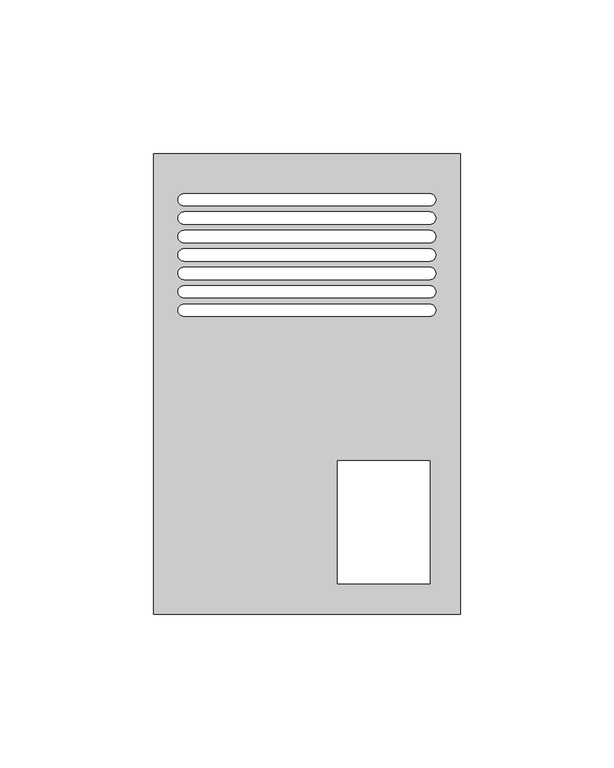
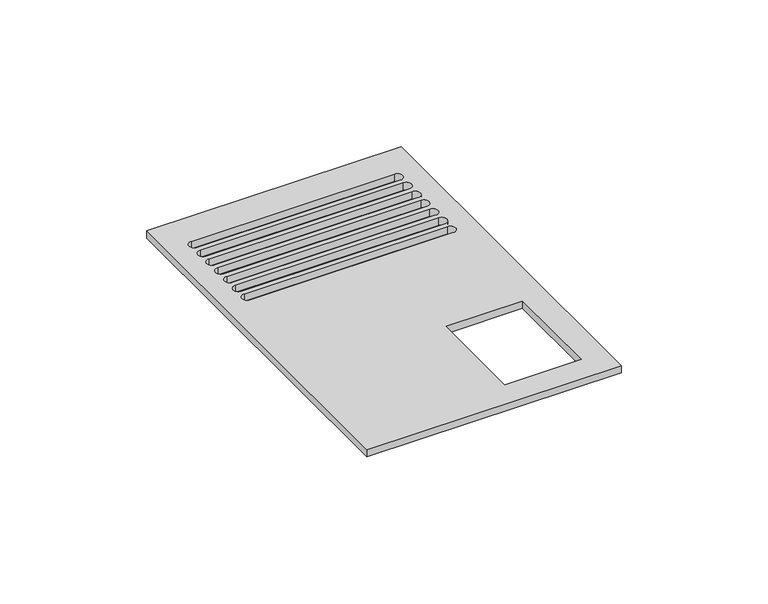
"""IFC4 building model written with IfcOpenShell, lengths in millimetres: proxy geometry, TSP Intercom Point : TSP Intercom Point."""

from ifc_helpers import new_model, si_unit, point, frame_2d, origin, origin_with_axes, place, context, project, spatial, polyline, circle_curve, trimmed, segment, composite_curve, outline, extrude, source, transform, mapped, element, save


def electrical_fixtures_fec92b32(model_context):
    return source(origin(), model_context, "Body", "SweptSolid", [
        extrude(outline(polyline([(-100.0, 75.0), (0.0, 75.0), (0.0, -75.0), (-100.0, -75.0), (-100.0, 75.0)]), holes=[polyline([(-40.0, -65.0), (-10.0, -65.0), (-10.0, -25.0), (-40.0, -25.0), (-40.0, -65.0)]), composite_curve([segment(polyline([(-10.0, 62.0), (-90.0, 62.0)]), True, "CONTINUOUS"), segment(trimmed(circle_curve(frame_2d((-90.0, 60.0)), 2.0), [point((-90.0, 62.0))], [point((-90.0, 58.0))], True, "CARTESIAN"), True, "CONTINUOUS"), segment(polyline([(-90.0, 58.0), (-10.0, 58.0)]), True, "CONTINUOUS"), segment(trimmed(circle_curve(frame_2d((-10.0, 60.0)), 2.0), [point((-10.0, 58.0))], [point((-10.0, 62.0))], True, "CARTESIAN"), True, "CONTINUOUS")], self_intersect=False), composite_curve([segment(polyline([(-10.0, 56.0), (-90.0, 56.0)]), True, "CONTINUOUS"), segment(trimmed(circle_curve(frame_2d((-90.0, 54.0)), 2.0), [point((-90.0, 56.0))], [point((-90.0, 52.0))], True, "CARTESIAN"), True, "CONTINUOUS"), segment(polyline([(-90.0, 52.0), (-10.0, 52.0)]), True, "CONTINUOUS"), segment(trimmed(circle_curve(frame_2d((-10.0, 54.0)), 2.0), [point((-10.0, 52.0))], [point((-10.0, 56.0))], True, "CARTESIAN"), True, "CONTINUOUS")], self_intersect=False), composite_curve([segment(polyline([(-10.0, 50.0), (-90.0, 50.0)]), True, "CONTINUOUS"), segment(trimmed(circle_curve(frame_2d((-90.0, 48.0)), 2.0), [point((-90.0, 50.0))], [point((-90.0, 46.0))], True, "CARTESIAN"), True, "CONTINUOUS"), segment(polyline([(-90.0, 46.0), (-10.0, 46.0)]), True, "CONTINUOUS"), segment(trimmed(circle_curve(frame_2d((-10.0, 48.0)), 2.0), [point((-10.0, 46.0))], [point((-10.0, 50.0))], True, "CARTESIAN"), True, "CONTINUOUS")], self_intersect=False), composite_curve([segment(polyline([(-10.0, 44.0), (-90.0, 44.0)]), True, "CONTINUOUS"), segment(trimmed(circle_curve(frame_2d((-90.0, 42.0)), 2.0), [point((-90.0, 44.0))], [point((-90.0, 40.0))], True, "CARTESIAN"), True, "CONTINUOUS"), segment(polyline([(-90.0, 40.0), (-10.0, 40.0)]), True, "CONTINUOUS"), segment(trimmed(circle_curve(frame_2d((-10.0, 42.0)), 2.0), [point((-10.0, 40.0))], [point((-10.0, 44.0))], True, "CARTESIAN"), True, "CONTINUOUS")], self_intersect=False), composite_curve([segment(polyline([(-10.0, 38.0), (-90.0, 38.0)]), True, "CONTINUOUS"), segment(trimmed(circle_curve(frame_2d((-90.0, 36.0)), 2.0), [point((-90.0, 38.0))], [point((-90.0, 34.0))], True, "CARTESIAN"), True, "CONTINUOUS"), segment(polyline([(-90.0, 34.0), (-10.0, 34.0)]), True, "CONTINUOUS"), segment(trimmed(circle_curve(frame_2d((-10.0, 36.0)), 2.0), [point((-10.0, 34.0))], [point((-10.0, 38.0))], True, "CARTESIAN"), True, "CONTINUOUS")], self_intersect=False), composite_curve([segment(polyline([(-10.0, 32.0), (-90.0, 32.0)]), True, "CONTINUOUS"), segment(trimmed(circle_curve(frame_2d((-90.0, 30.0)), 2.0), [point((-90.0, 32.0))], [point((-90.0, 28.0))], True, "CARTESIAN"), True, "CONTINUOUS"), segment(polyline([(-90.0, 28.0), (-10.0, 28.0)]), True, "CONTINUOUS"), segment(trimmed(circle_curve(frame_2d((-10.0, 30.0)), 2.0), [point((-10.0, 28.0))], [point((-10.0, 32.0))], True, "CARTESIAN"), True, "CONTINUOUS")], self_intersect=False), composite_curve([segment(polyline([(-10.0, 26.0), (-90.0, 26.0)]), True, "CONTINUOUS"), segment(trimmed(circle_curve(frame_2d((-90.0, 24.0)), 2.0), [point((-90.0, 26.0))], [point((-90.0, 22.0))], True, "CARTESIAN"), True, "CONTINUOUS"), segment(polyline([(-90.0, 22.0), (-10.0, 22.0)]), True, "CONTINUOUS"), segment(trimmed(circle_curve(frame_2d((-10.0, 24.0)), 2.0), [point((-10.0, 22.0))], [point((-10.0, 26.0))], True, "CARTESIAN"), True, "CONTINUOUS")], self_intersect=False)]), origin_with_axes(), (0.0, 0.0, 1.0), 3.0),
    ])


if __name__ == "__main__":
    model = new_model("IFC4")
    model_context = context("Model", 3, world=origin())
    ifc_project = project(units=[si_unit("LENGTHUNIT", "METRE", prefix="MILLI")], contexts=[model_context])
    site = spatial("IfcSite", under=ifc_project)
    building = spatial("IfcBuilding", under=site)
    placement = place(None, origin())
    electrical_fixtures_shape = electrical_fixtures_fec92b32(model_context)
    element("IfcBuildingElementProxy", 1, Name="TSP Intercom Point : TSP Intercom Point", ObjectType="TSP Intercom Point : TSP Intercom Point", at=placement, inside=building, context=model_context, shape_type="MappedRepresentation", body=[
        mapped(electrical_fixtures_shape, transform((0.0, 0.0, 0.0), x_axis=(1.0, 0.0, 0.0), y_axis=(0.0, 1.0, 0.0), z_axis=(0.0, 0.0, 1.0))),
    ])
    save(model, "model.ifc")

# Revit data of these elements
# Type "TSP Intercom Point : TSP Intercom Point"
#   Model = "TSP_ELECEGIP"
#   Default Elevation = 0
# Element 1 (IfcBuildingElementProxy, "TSP Intercom Point : TSP Intercom Point")
#   Materials on its faces: "Plastic, Opaque Black"
# Materials
#   "Plastic, Opaque Black": class "Plastic", colour RGB 0 0 0, transparency 0.7, Description = "Plastic, generic, opaque black", Cost = 0
